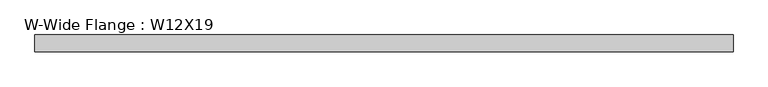
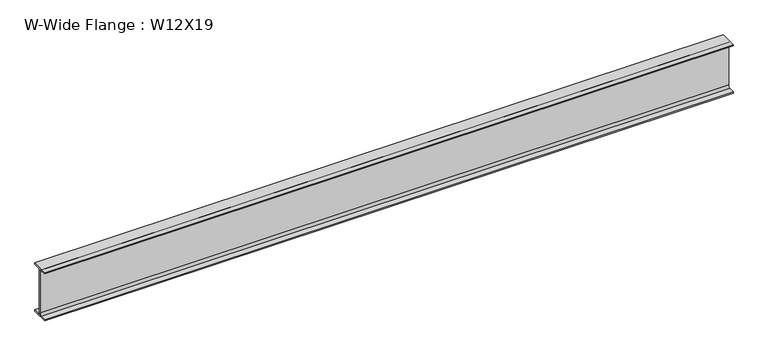
"""IFC4 building model written with IfcOpenShell, lengths in millimetres: beam geometry, W-Wide Flange : W12X19."""

from ifc_helpers import new_model, si_unit, point, frame, frame_2d, origin, place, context, project, spatial, polyline, circle_curve, trimmed, segment, composite_curve, outline, extrude, source, transform, mapped, element, save


def w_wide_flange_w12x19_0333fea9(model_context):
    return source(origin(), model_context, "Body", "SweptSolid", [
        extrude(outline(composite_curve([segment(polyline([(50.927, -146.05), (50.927, -154.94), (-50.927, -154.94), (-50.927, -146.05), (-16.3195, -146.05)]), True, "CONTINUOUS"), segment(trimmed(circle_curve(frame_2d((-16.3195, -132.715)), 13.335), [point((-16.3195, -146.05))], [point((-2.9845, -132.715))], True, "CARTESIAN"), True, "CONTINUOUS"), segment(polyline([(-2.9845, -132.715), (-2.9845, 132.715)]), True, "CONTINUOUS"), segment(trimmed(circle_curve(frame_2d((-16.3195, 132.715)), 13.335), [point((-2.9845, 132.715))], [point((-16.3195, 146.05))], True, "CARTESIAN"), True, "CONTINUOUS"), segment(polyline([(-16.3195, 146.05), (-50.927, 146.05), (-50.927, 154.94), (50.927, 154.94), (50.927, 146.05), (16.3195, 146.05)]), True, "CONTINUOUS"), segment(trimmed(circle_curve(frame_2d((16.3195, 132.715)), 13.335), [point((16.3195, 146.05))], [point((2.9845, 132.715))], True, "CARTESIAN"), True, "CONTINUOUS"), segment(polyline([(2.9845, 132.715), (2.9845, -132.715)]), True, "CONTINUOUS"), segment(trimmed(circle_curve(frame_2d((16.3195, -132.715)), 13.335), [point((2.9845, -132.715))], [point((16.3195, -146.05))], True, "CARTESIAN"), True, "CONTINUOUS"), segment(polyline([(16.3195, -146.05), (50.927, -146.05)]), True, "CONTINUOUS")], self_intersect=False)), frame((-2082.8, 0.0, 0.0), z_axis=(1.0, 0.0, 0.0), x_axis=(0.0, 1.0, 0.0)), (0.0, 0.0, 1.0), 4165.6),
    ])


if __name__ == "__main__":
    model = new_model("IFC4")
    model_context = context("Model", 3, world=origin())
    ifc_project = project(units=[si_unit("LENGTHUNIT", "METRE", prefix="MILLI")], contexts=[model_context])
    site = spatial("IfcSite", under=ifc_project)
    building = spatial("IfcBuilding", under=site)
    placement = place(None, origin())
    w_wide_flange_w12x19_shape = w_wide_flange_w12x19_0333fea9(model_context)
    element("IfcBeam", 1, ObjectType="W-Wide Flange : W12X19", at=placement, inside=building, context=model_context, shape_type="MappedRepresentation", body=[
        mapped(w_wide_flange_w12x19_shape, transform((0.0, 0.0, 0.0), x_axis=(1.0, 0.0, 0.0), y_axis=(0.0, 1.0, 0.0), z_axis=(0.0, 0.0, 1.0))),
    ])
    save(model, "model.ifc")

# Revit data of these elements
# Type "W-Wide Flange : W12X19"
#   Assembly Code = "B10"
#   W = 19
#   Length [instance default] = 5' - 0"
#   bf = 0' - 4.01"
#   d = 1' - 0.2"
#   k = 0' - 0 7/8"
#   k2 = 0' - 0.525"
#   tf = 0' - 0.35"
#   tw = 0' - 0.235"
#   A = 0.0386806 SF
#   Structural Material [instance default] = Steel ASTM A992
# Element 1 (IfcBeam, "W-Wide Flange : W12X19")
#   Materials on its faces: "Steel ASTM A992"
# Materials
#   "Steel ASTM A992": class "Metal", colour RGB 199 199 199, transparency 0, Description = "Structural steel 50ksi", Cost = 0
